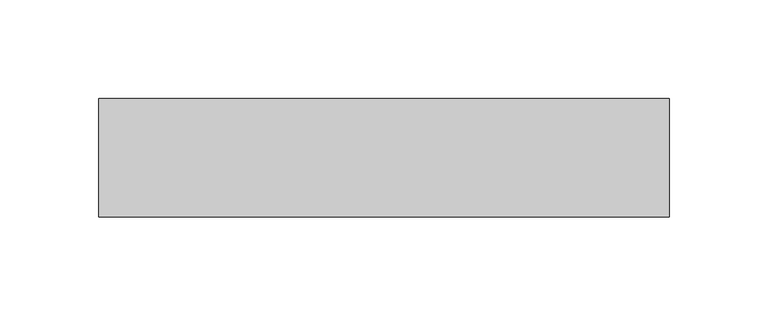
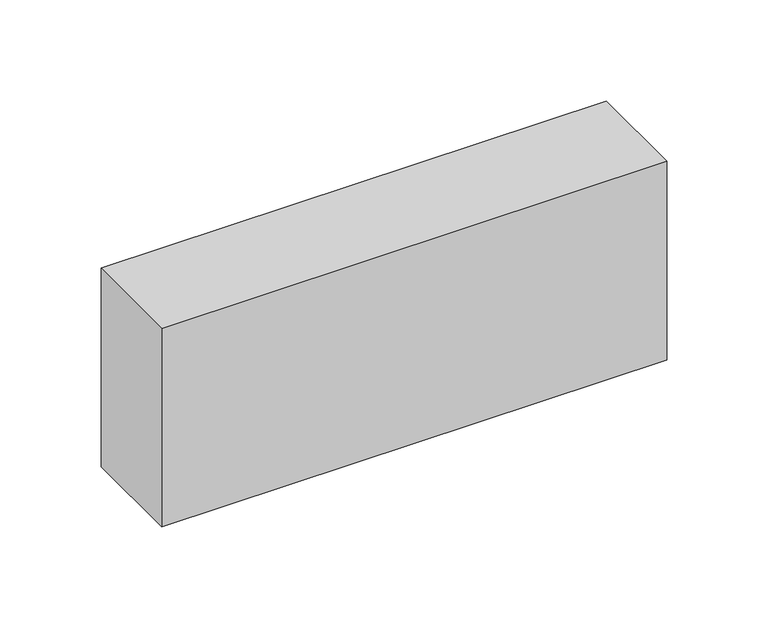
"""IFC4 building model written with IfcOpenShell, lengths in millimetres: beam geometry, Madeira de lei : Berço 6x12cm."""

from ifc_helpers import new_model, si_unit, frame, origin, place, context, project, spatial, polyline, outline, extrude, source, transform, mapped, element, save


def beam_e1aa0c85(model_context):
    return source(origin(), model_context, "Body", "SweptSolid", [
        extrude(outline(polyline([(144.2686794, 30.0), (144.2686794, -30.0), (-144.2686794, -30.0), (-144.2686794, 30.0), (144.2686794, 30.0)])), frame((0.0, 0.0, -60.0), z_axis=(0.0, 0.0, 1.0), x_axis=(1.0, 0.0, 0.0)), (0.0, 0.0, 1.0), 120.0),
    ])


if __name__ == "__main__":
    model = new_model("IFC4")
    model_context = context("Model", 3, world=origin())
    ifc_project = project(units=[si_unit("LENGTHUNIT", "METRE", prefix="MILLI")], contexts=[model_context])
    site = spatial("IfcSite", under=ifc_project)
    building = spatial("IfcBuilding", under=site)
    placement = place(None, origin())
    beam_shape = beam_e1aa0c85(model_context)
    element("IfcBeam", 1, ObjectType="Madeira de lei : Berço 6x12cm", at=placement, inside=building, context=model_context, shape_type="MappedRepresentation", body=[
        mapped(beam_shape, transform((0.0, 0.0, 0.0), x_axis=(1.0, 0.0, 0.0), y_axis=(0.0, 1.0, 0.0), z_axis=(0.0, 0.0, 1.0))),
    ])
    save(model, "model.ifc")

# Revit data of these elements
# Type "Madeira de lei : Berço 6x12cm"
#   A = 0.02 m²
#   Length [instance default] = 1.524 m
#   b = 0.06 m
#   d = 0.12 m
#   Structural Material [instance default] = none
#   Assembly Code = ""
# Element 1 (IfcBeam, "Madeira de lei : Berço 6x12cm")
#   Structural Material = .MADEIRAMENTO
#   Materials on its faces: ".MADEIRAMENTO"
# Materials
#   ".MADEIRAMENTO": class ".CC_MADEIRAS", colour RGB 212 179 113, transparency 0, Cost = 0
